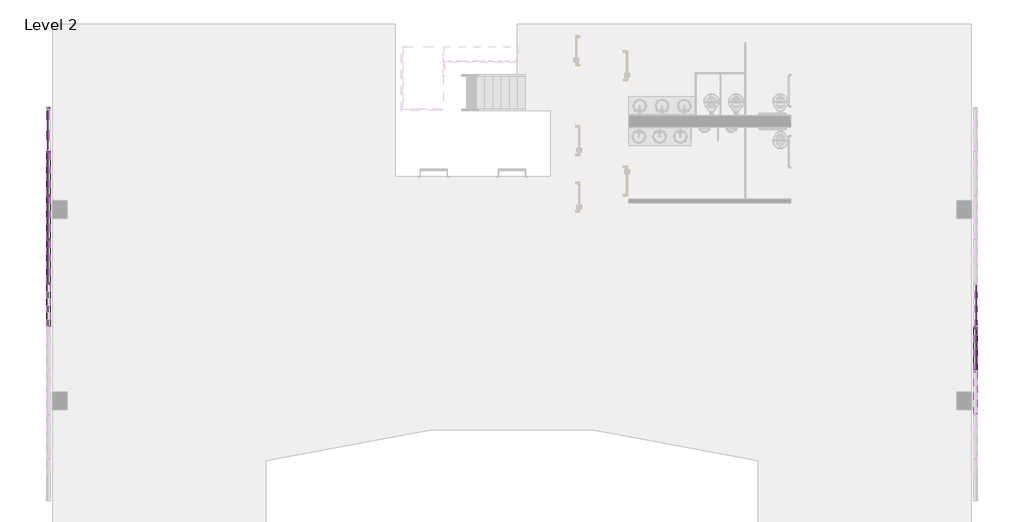
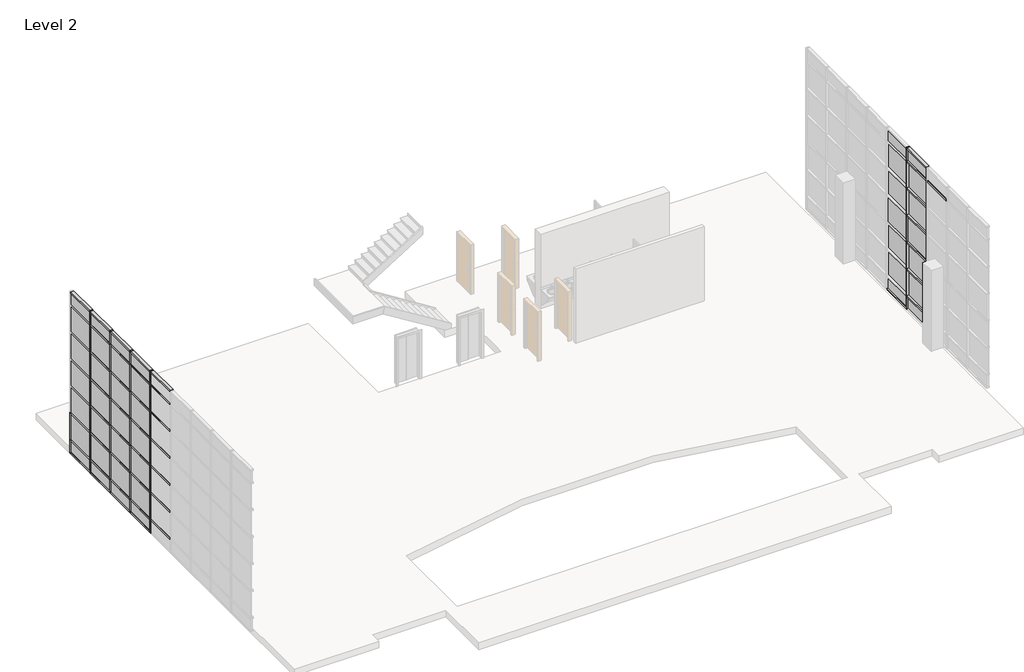
# One storey, part 4 of 6: 79 members, 42 plates.
# Revit data of these elements (continued)
# Room at (601.881, 5531.589) mm, phase "New Construction", upper level "Level 2", upper offset 8' - 0", lower offset 0' - 0" (continued)
#   Number = "206"
#   Name = "Elec"
# Room at (601.881, 3635.746) mm, phase "New Construction", upper level "Level 2", upper offset 8' - 0", lower offset 0' - 0"
#   Number = "207"
#   Name = "Mech"
# Room at (-2043.483, 5531.589) mm, phase "New Construction", upper level "Level 2", upper offset 8' - 0", lower offset 0' - 0"
#   Number = "208"
#   Name = "Elevator"
